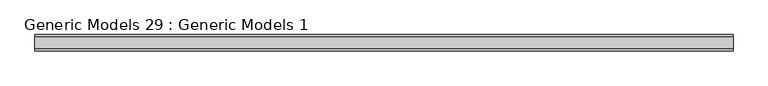
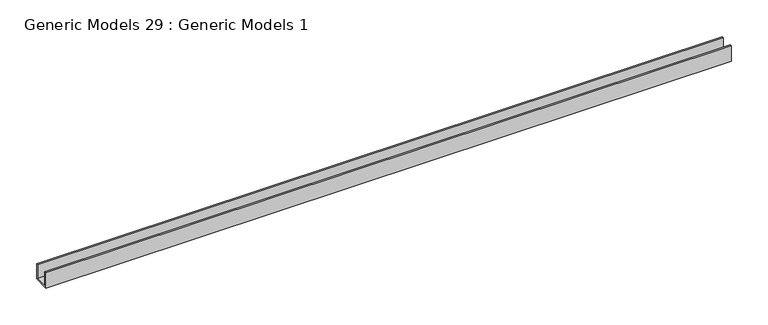
"""IFC4 building model written with IfcOpenShell, lengths in millimetres: proxy geometry, Generic Models 29 : Generic Models 1."""

from ifc_helpers import new_model, si_unit, frame, origin, place, context, project, spatial, polyline, outline, extrude, source, transform, mapped, element, save


def generic_models_29_generic_models_1_1f362c28(model_context):
    return source(origin(), model_context, "Body", "SweptSolid", [
        extrude(outline(polyline([(39527.9428995, 0.0), (39502.5428995, 0.0), (39502.5428995, 25.4), (39505.7178995, 25.4), (39505.7178995, 3.175), (39524.7678995, 3.175), (39524.7678995, 25.4), (39527.9428995, 25.4), (39527.9428995, 0.0)])), frame((51499.3577305, 0.0, 0.0), z_axis=(1.0, 0.0, 0.0), x_axis=(0.0, 1.0, 0.0)), (0.0, 0.0, 1.0), 1079.5),
    ])


if __name__ == "__main__":
    model = new_model("IFC4")
    model_context = context("Model", 3, world=origin())
    ifc_project = project(units=[si_unit("LENGTHUNIT", "METRE", prefix="MILLI")], contexts=[model_context])
    site = spatial("IfcSite", under=ifc_project)
    building = spatial("IfcBuilding", under=site)
    placement = place(None, origin())
    generic_models_29_generic_models_1_shape = generic_models_29_generic_models_1_1f362c28(model_context)
    element("IfcBuildingElementProxy", 1, Name="Generic Models 29 : Generic Models 1", ObjectType="Generic Models 29 : Generic Models 1", at=placement, inside=building, context=model_context, shape_type="MappedRepresentation", body=[
        mapped(generic_models_29_generic_models_1_shape, transform((0.0, 0.0, 0.0), x_axis=(1.0, 0.0, 0.0), y_axis=(0.0, 1.0, 0.0), z_axis=(0.0, 0.0, 1.0))),
    ])
    save(model, "model.ifc")

# Revit data of these elements
# Element 1 (IfcBuildingElementProxy, "Generic Models 29 : Generic Models 1")
#   Materials on its faces: "ALUM. SILL PROFILE TO MATCH EXISTING AT TENANT ENTRANCE"
# Materials
#   "ALUM. SILL PROFILE TO MATCH EXISTING AT TENANT ENTRANCE": class "Unassigned", colour RGB 226 225 224, transparency 0, Cost = 0
